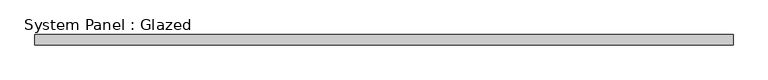
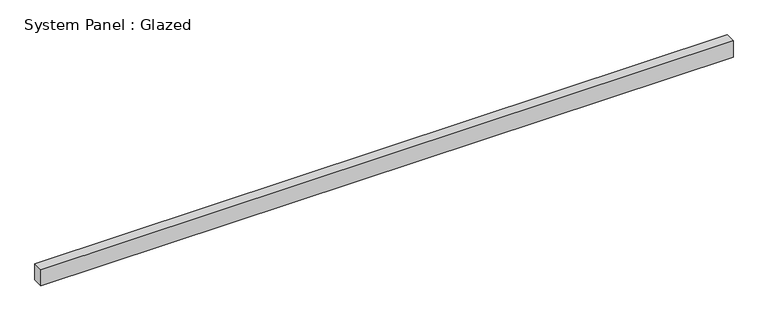
"""IFC4 building model written with IfcOpenShell, lengths in millimetres: plate geometry, System Panel : Glazed."""

import ifcopenshell
import ifcopenshell.guid

model = None  # the IFC model being written
_history = None  # IfcOwnerHistory: only IFC2X3 demands one
_inside = {}  # id of a spatial element -> (the spatial element, [elements in it])
_under = {}  # id of a project, library or spatial element -> (it, [spatial elements below it])
_declared = {}  # id of a project -> (the project, [libraries it declares])
_typed = {}  # id of a type object -> (the type object, [elements of that type])
_made_of = {}  # id of a material, layer set ... -> (it, [elements and type objects made of it])


def new_model(schema):
    """Start an empty IFC model of exactly this schema.

    Asked for "IFC4X3", IfcOpenShell would pick the latest addendum, in which some entities
    have other attributes; the version numbers below select the first issue.
    IFC2X3 requires an IfcOwnerHistory on every rooted entity: one is made here for all.
    """
    global model, _history
    if schema == "IFC4X3":
        model = ifcopenshell.file(schema_version=(4, 3, 0, 0))
    else:
        model = ifcopenshell.file(schema=schema)
    _inside.clear()
    _under.clear()
    _declared.clear()
    _typed.clear()
    _made_of.clear()
    _history = None
    if model.schema == "IFC2X3":
        org = make("IfcOrganization", Name="unknown")
        user = make(
            "IfcPersonAndOrganization",
            ThePerson=make("IfcPerson", FamilyName="unknown"),
            TheOrganization=org,
        )
        app = make(
            "IfcApplication",
            ApplicationDeveloper=org,
            Version="unknown",
            ApplicationFullName="unknown",
            ApplicationIdentifier="unknown",
        )
        _history = make(
            "IfcOwnerHistory",
            OwningUser=user,
            OwningApplication=app,
            ChangeAction="ADDED",
            CreationDate=0,
        )
    return model


def make(cls, **values):
    """One entity of the class cls with the attributes given. An attribute that is None is left unset."""
    return model.create_entity(
        cls, **{name: value for name, value in values.items() if value is not None}
    )


def rooted(cls, **values):
    """An entity with a GlobalId (a new one), such as an element, a storey or a relation."""
    return make(cls, GlobalId=ifcopenshell.guid.new(), OwnerHistory=_history, **values)


def si_unit(unit_type, name, prefix=None):
    """IfcSIUnit, for example si_unit("LENGTHUNIT", "METRE", prefix="MILLI")."""
    return make("IfcSIUnit", UnitType=unit_type, Prefix=prefix, Name=name)


def assignment(units):
    """IfcUnitAssignment: the units of a project."""
    return None if units is None else make("IfcUnitAssignment", Units=units)


def point(xyz):
    """IfcCartesianPoint."""
    return None if xyz is None else make("IfcCartesianPoint", Coordinates=xyz)


def direction(xyz):
    """IfcDirection."""
    return None if xyz is None else make("IfcDirection", DirectionRatios=xyz)


def frame(location, z_axis=None, x_axis=None):
    """IfcAxis2Placement3D, a coordinate frame: its origin and axes. An axis left out is left unset."""
    return make(
        "IfcAxis2Placement3D",
        Location=point(location),
        Axis=direction(z_axis),
        RefDirection=direction(x_axis),
    )


def origin():
    """The frame at (0, 0, 0) with its axes left unset."""
    return frame((0.0, 0.0, 0.0))


def origin_with_axes():
    """The frame at (0, 0, 0) with the z axis (0, 0, 1) and the x axis (1, 0, 0) written out."""
    return frame((0.0, 0.0, 0.0), z_axis=(0.0, 0.0, 1.0), x_axis=(1.0, 0.0, 0.0))


def place(relative_to, where):
    """IfcLocalPlacement: puts the frame where relative to a parent placement (None: the world)."""
    return make(
        "IfcLocalPlacement", PlacementRelTo=relative_to, RelativePlacement=where
    )


def context(
    kind, dimensions, precision=None, world=None, true_north=None, identifier=None
):
    """IfcGeometricRepresentationContext, for example the 3D "Model" context."""
    return make(
        "IfcGeometricRepresentationContext",
        ContextIdentifier=identifier,
        ContextType=kind,
        CoordinateSpaceDimension=dimensions,
        Precision=precision,
        WorldCoordinateSystem=world,
        TrueNorth=true_north,
    )


def project(units=None, contexts=None):
    """IfcProject with its units and contexts."""
    return rooted(
        "IfcProject",
        Name="project",
        RepresentationContexts=contexts,
        UnitsInContext=assignment(units),
    )


def spatial(cls, under=None, at=None, **own):
    """A site, building, storey or space (cls), placed at a placement, below another one or the project."""
    s = rooted(cls, ObjectPlacement=at, **own)
    if under is not None:
        _under.setdefault(under.id(), (under, []))[1].append(s)
    return s


def polyline(points):
    """IfcPolyline through the points."""
    return make("IfcPolyline", Points=[point(p) for p in points])


def outline(outer, holes=None, kind="AREA"):
    """IfcArbitraryClosedProfileDef: a profile drawn as a closed curve; with holes, ...WithVoids."""
    if holes is None:
        return make("IfcArbitraryClosedProfileDef", ProfileType=kind, OuterCurve=outer)
    return make(
        "IfcArbitraryProfileDefWithVoids",
        ProfileType=kind,
        OuterCurve=outer,
        InnerCurves=holes,
    )


def extrude(swept, where, along, depth):
    """IfcExtrudedAreaSolid: the profile swept, set in the frame where, extruded along a direction by depth."""
    return make(
        "IfcExtrudedAreaSolid",
        SweptArea=swept,
        Position=where,
        ExtrudedDirection=direction(along),
        Depth=depth,
    )


def shape(context_of_items, identifier, shape_type, items):
    """IfcShapeRepresentation: the items that make up one representation, for example the "Body"."""
    return make(
        "IfcShapeRepresentation",
        ContextOfItems=context_of_items,
        RepresentationIdentifier=identifier,
        RepresentationType=shape_type,
        Items=items,
    )


def source(mapping_origin, context_of_items, identifier, shape_type, items):
    """IfcRepresentationMap: a shape defined once, which mapped items show again and again."""
    return make(
        "IfcRepresentationMap",
        MappingOrigin=mapping_origin,
        MappedRepresentation=shape(context_of_items, identifier, shape_type, items),
    )


def transform(
    local_origin,
    x_axis=None,
    y_axis=None,
    z_axis=None,
    scale=None,
    scale2=None,
    scale3=None,
    uniform=True,
):
    """IfcCartesianTransformationOperator3D, or its non-uniform kind. x_axis, y_axis, z_axis: its Axis1, 2, 3."""
    if uniform:
        return make(
            "IfcCartesianTransformationOperator3D",
            Axis1=direction(x_axis),
            Axis2=direction(y_axis),
            LocalOrigin=point(local_origin),
            Scale=scale,
            Axis3=direction(z_axis),
        )
    return make(
        "IfcCartesianTransformationOperator3DnonUniform",
        Axis1=direction(x_axis),
        Axis2=direction(y_axis),
        LocalOrigin=point(local_origin),
        Scale=scale,
        Axis3=direction(z_axis),
        Scale2=scale2,
        Scale3=scale3,
    )


def mapped(mapping_source, mapping_target):
    """IfcMappedItem: shows the shape of a source again, moved by a transform."""
    return make(
        "IfcMappedItem", MappingSource=mapping_source, MappingTarget=mapping_target
    )


def made_of(thing, what):
    """Note that an element or type object is made of a material, layer set ...; save() writes the relation."""
    if what is not None:
        _made_of.setdefault(what.id(), (what, []))[1].append(thing)
    return thing


def element(
    cls,
    number,
    at=None,
    inside=None,
    cuts=None,
    type_object=None,
    material=None,
    context=None,
    identifier="Body",
    shape_type=None,
    held_by="IfcProductDefinitionShape",
    body=None,
    shapes=None,
    **own,
):
    """One element of the class cls, such as IfcWall. Its Tag is "e" and its number.

    at: its placement. inside: the storey or other place that contains it. cuts: it is an
    opening in that element (IfcRelVoidsElement). A single representation is given by context,
    identifier, shape_type and body (its items); several are given by shapes. held_by: the class
    of the entity that holds the representations. save() writes the other relations.
    """
    e = rooted(cls, Tag="e%d" % number, ObjectPlacement=at, **own)
    if body is not None:
        shapes = [shape(context, identifier, shape_type, body)]
    if shapes is not None:
        e.Representation = make(held_by, Representations=shapes)
    if inside is not None:
        _inside.setdefault(inside.id(), (inside, []))[1].append(e)
    if cuts is not None:
        rooted(
            "IfcRelVoidsElement", RelatingBuildingElement=cuts, RelatedOpeningElement=e
        )
    if type_object is not None:
        _typed.setdefault(type_object.id(), (type_object, []))[1].append(e)
    return made_of(e, material)


def aggregate(whole, parts):
    """IfcRelAggregates: a whole, such as a stair, and the parts it consists of."""
    return rooted("IfcRelAggregates", RelatingObject=whole, RelatedObjects=parts)


def save(model, path):
    """Write the relations noted so far, then the file.

    IfcRelAggregates (storeys below a building ...), IfcRelContainedInSpatialStructure (elements
    in a storey), IfcRelDefinesByType, IfcRelAssociatesMaterial and IfcRelDeclares: one each for
    every whole, place, type object, material and project.
    """
    for whole, parts in _under.values():
        aggregate(whole, parts)
    for where, things in _inside.values():
        rooted(
            "IfcRelContainedInSpatialStructure",
            RelatedElements=things,
            RelatingStructure=where,
        )
    for kind, things in _typed.values():
        rooted("IfcRelDefinesByType", RelatedObjects=things, RelatingType=kind)
    for what, things in _made_of.values():
        rooted("IfcRelAssociatesMaterial", RelatedObjects=things, RelatingMaterial=what)
    for by, libraries in _declared.values():
        rooted("IfcRelDeclares", RelatingContext=by, RelatedDefinitions=libraries)
    model.write(path)


def system_panel_glazed_8b4ddac8(model_context):
    return source(origin(), model_context, "Body", "SweptSolid", [
        extrude(outline(polyline([(838.2000002, -44.45), (-838.2000002, -44.45), (-838.2000002, -19.05), (838.2000002, -19.05), (838.2000002, -44.45)])), origin_with_axes(), (0.0, 0.0, 1.0), 41.9143134),
    ])


if __name__ == "__main__":
    model = new_model("IFC4")
    model_context = context("Model", 3, world=origin())
    ifc_project = project(units=[si_unit("LENGTHUNIT", "METRE", prefix="MILLI")], contexts=[model_context])
    site = spatial("IfcSite", under=ifc_project)
    building = spatial("IfcBuilding", under=site)
    placement = place(None, origin())
    system_panel_glazed_shape = system_panel_glazed_8b4ddac8(model_context)
    element("IfcPlate", 1, ObjectType="System Panel : Glazed", at=placement, inside=building, context=model_context, shape_type="MappedRepresentation", body=[
        mapped(system_panel_glazed_shape, transform((0.0, 0.0, 0.0), x_axis=(1.0, 0.0, 0.0), y_axis=(0.0, 1.0, 0.0), z_axis=(0.0, 0.0, 1.0))),
    ])
    save(model, "model.ifc")

# Revit data of these elements
# Type "System Panel : Glazed"
#   Construction Type Id = "GSP4R"
#   Analytic Construction = "1/8 in Pilkington single glazing"
#   Visual Light Transmittance = 0.9
#   Solar Heat Gain Coefficient = 0.86
#   Heat Transfer Coefficient (U) = 1.18115 BTU/(h·ft²·°F)
#   Define Thermal Properties by = 1
# Element 1 (IfcPlate, "System Panel : Glazed")
#   Materials on its faces: "Glass"
# Materials
#   "Glass": class "Glass", colour RGB 0 128 192, transparency 0.75, Description = "Soda Lime Glass", Cost = 0
